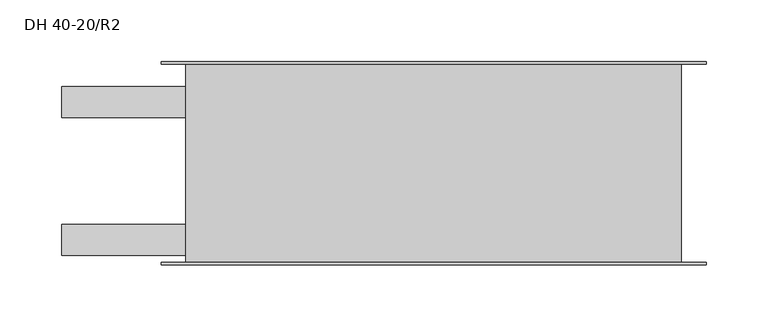
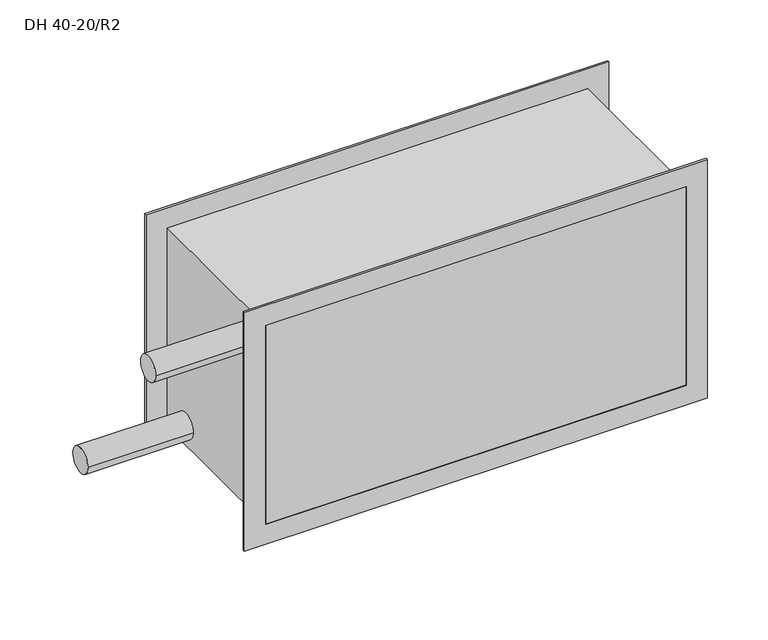
"""IFC4 building model written with IfcOpenShell, lengths in millimetres: proxy geometry, Воздухонагреватель водяной DH : DH 40-20/R2."""

from ifc_helpers import new_model, si_unit, point, frame, frame_2d, origin, place, context, project, spatial, polyline, circle_curve, trimmed, segment, composite_curve, outline, extrude, source, transform, mapped, element, save


def dh_40_20_r2_a288613b(model_context):
    return source(origin(), model_context, "Body", "SweptSolid", [
        extrude(outline(composite_curve([segment(trimmed(circle_curve(frame_2d((-62.0, 80.0)), 12.5), [point((-74.5, 80.0))], [point((-49.5, 80.0))], False, "CARTESIAN"), True, "CONTINUOUS"), segment(trimmed(circle_curve(frame_2d((-62.0, 80.0)), 12.5), [point((-49.5, 80.0))], [point((-74.5, 80.0))], False, "CARTESIAN"), True, "CONTINUOUS")], self_intersect=False)), frame((-300.0, 0.0, 0.0), z_axis=(1.0, 0.0, 0.0), x_axis=(0.0, 1.0, 0.0)), (0.0, 0.0, 1.0), 100.0),
        extrude(outline(composite_curve([segment(trimmed(circle_curve(frame_2d((49.5, -80.0)), 12.5), [point((37.0, -80.0))], [point((62.0, -80.0))], False, "CARTESIAN"), True, "CONTINUOUS"), segment(trimmed(circle_curve(frame_2d((49.5, -80.0)), 12.5), [point((62.0, -80.0))], [point((37.0, -80.0))], False, "CARTESIAN"), True, "CONTINUOUS")], self_intersect=False)), frame((-300.0, 0.0, 0.0), z_axis=(1.0, 0.0, 0.0), x_axis=(0.0, 1.0, 0.0)), (0.0, 0.0, 1.0), 100.0),
        extrude(outline(polyline([(120.0, 220.0), (120.0, -220.0), (-120.0, -220.0), (-120.0, 220.0), (120.0, 220.0)]), holes=[polyline([(-100.0, 200.0), (-100.0, -200.0), (100.0, -200.0), (100.0, 200.0), (-100.0, 200.0)])]), frame((0.0, 80.0, 0.0), z_axis=(0.0, 1.0, 0.0), x_axis=(0.0, 0.0, 1.0)), (0.0, 0.0, 1.0), 2.0),
        extrude(outline(polyline([(120.0, -220.0), (-120.0, -220.0), (-120.0, 220.0), (120.0, 220.0), (120.0, -220.0)]), holes=[polyline([(100.0, 200.0), (-100.0, 200.0), (-100.0, -200.0), (100.0, -200.0), (100.0, 200.0)])]), frame((0.0, -82.0, 0.0), z_axis=(0.0, 1.0, 0.0), x_axis=(0.0, 0.0, 1.0)), (0.0, 0.0, 1.0), 2.0),
        extrude(outline(polyline([(200.0, -82.0), (-200.0, -82.0), (-200.0, 82.0), (200.0, 82.0), (200.0, -82.0)])), frame((0.0, 0.0, -100.0), z_axis=(0.0, 0.0, 1.0), x_axis=(1.0, 0.0, 0.0)), (0.0, 0.0, 1.0), 200.0),
    ])


if __name__ == "__main__":
    model = new_model("IFC4")
    model_context = context("Model", 3, world=origin())
    ifc_project = project(units=[si_unit("LENGTHUNIT", "METRE", prefix="MILLI")], contexts=[model_context])
    site = spatial("IfcSite", under=ifc_project)
    building = spatial("IfcBuilding", under=site)
    placement = place(None, origin())
    dh_40_20_r2_shape = dh_40_20_r2_a288613b(model_context)
    element("IfcBuildingElementProxy", 1, Name="Воздухонагреватель водяной DH : DH 40-20/R2", ObjectType="Воздухонагреватель водяной DH : DH 40-20/R2", at=placement, inside=building, context=model_context, shape_type="MappedRepresentation", body=[
        mapped(dh_40_20_r2_shape, transform((0.0, 0.0, 0.0), x_axis=(1.0, 0.0, 0.0), y_axis=(0.0, 1.0, 0.0), z_axis=(0.0, 0.0, 1.0))),
    ])
    save(model, "model.ifc")

# Revit data of these elements
# Type "Воздухонагреватель водяной DH : DH 40-20/R2"
#   Manufacturer = "WAER"
#   URL = "https://waer-air.com/"
#   ADSK_Система_Имя [instance default] = ""
#   ADSK_Наименование краткое = "DH 40-20/R2"
#   ADSK_Наименование = "Воздухонагреватель водяной DH 40-20/R2"
#   ADSK_Масса_Текст = "4.7"
#   ADSK_Марка = ""
#   ADSK_Код изделия = ""
#   ADSK_Завод-изготовитель = "WAER"
#   ADSK_Единица измерения = "шт."
#   ADSK_Расход воздуха = 0 m³/h
#   ADSK_Размер_Ширина = 400 mm
#   ADSK_Размер_Длина = 164 mm
#   ADSK_Размер_Диаметр = 25 mm
#   ADSK_Размер_Высота = 200 mm
#   ADSK_Потеря давления воздуха = 0.0 Pa
#   ADSK_Масса = 4.7
#   ADSK_Количество рядов = 2
#   ADSK_Количество = 1
#   Default Elevation = 0
#   Keynote = ""
